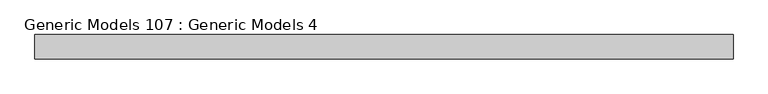
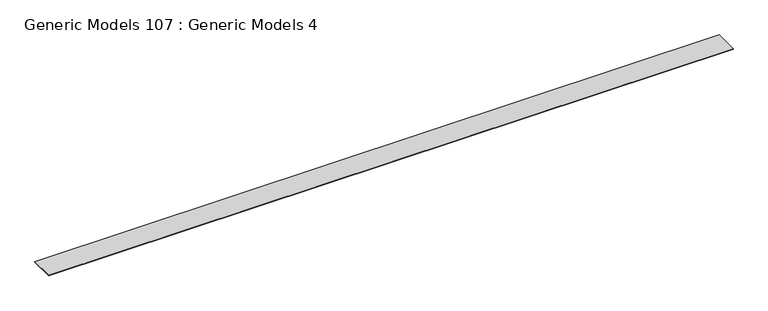
"""IFC4 building model written with IfcOpenShell, lengths in millimetres: proxy geometry, Generic Models 107 : Generic Models 4."""

from ifc_helpers import new_model, si_unit, frame, origin, place, context, project, spatial, polyline, outline, extrude, source, transform, mapped, element, save


def generic_models_107_generic_models_4_7de5214b(model_context):
    return source(origin(), model_context, "Body", "SweptSolid", [
        extrude(outline(polyline([(13598.6371921, 42937.689747), (13598.6371921, 42282.5431768), (-5044.9628079, 42282.5431768), (-5044.9628079, 42937.689747), (13598.6371921, 42937.689747)])), frame((0.0, 0.0, 126993.2559733), z_axis=(0.0, 0.0, 1.0), x_axis=(1.0, 0.0, 0.0)), (0.0, 0.0, 1.0), 19.05),
    ])


if __name__ == "__main__":
    model = new_model("IFC4")
    model_context = context("Model", 3, world=origin())
    ifc_project = project(units=[si_unit("LENGTHUNIT", "METRE", prefix="MILLI")], contexts=[model_context])
    site = spatial("IfcSite", under=ifc_project)
    building = spatial("IfcBuilding", under=site)
    placement = place(None, origin())
    generic_models_107_generic_models_4_shape = generic_models_107_generic_models_4_7de5214b(model_context)
    element("IfcBuildingElementProxy", 1, Name="Generic Models 107 : Generic Models 4", ObjectType="Generic Models 107 : Generic Models 4", at=placement, inside=building, context=model_context, shape_type="MappedRepresentation", body=[
        mapped(generic_models_107_generic_models_4_shape, transform((0.0, 0.0, 0.0), x_axis=(1.0, 0.0, 0.0), y_axis=(0.0, 1.0, 0.0), z_axis=(0.0, 0.0, 1.0))),
    ])
    save(model, "model.ifc")

# Revit data of these elements
# Element 1 (IfcBuildingElementProxy, "Generic Models 107 : Generic Models 4")
#   Materials on its faces: "_CDX PLYWOOD - SEE STRUCT DWGs"
# Materials
#   "_CDX PLYWOOD - SEE STRUCT DWGs": class "Generic", colour RGB 98 75 74, transparency 0, Cost = 0
